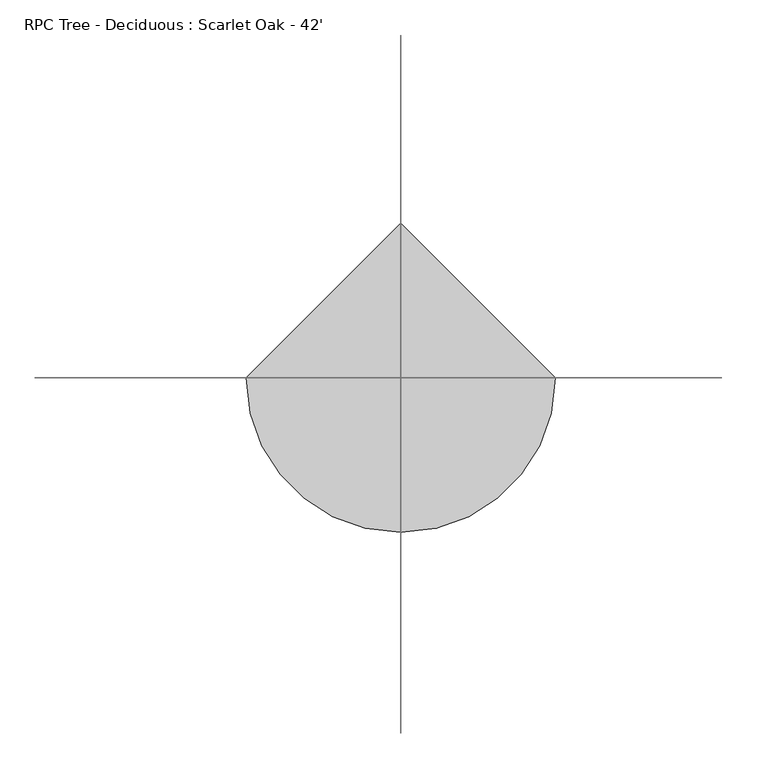
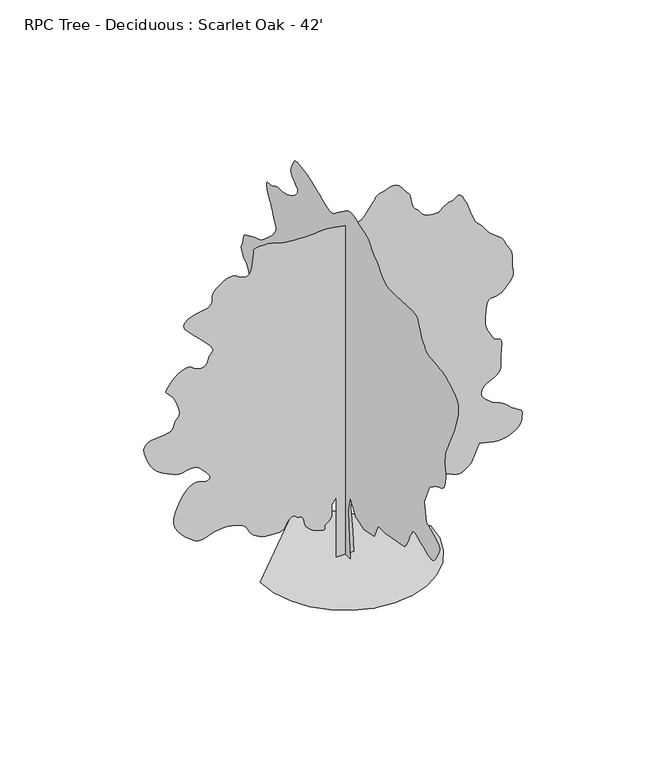
# IFC4 building model written with IfcOpenShell, lengths in millimetres: geographic element geometry, RPC Tree - Deciduous : Scarlet Oak - 42'.
# Revit data of these elements (continued)
# Type "RPC Tree - Deciduous : Scarlet Oak - 42'"
#   built-in parameter 1005198 = "{2, 15},{39, RPC-16-G0FB-J5PX-0LX6-U000-ST1L-LVER-AU},{1, 0},{1, 0},{2, 13},{1, 8},{5, Color},{1, 0},{1, 0},{3, 0.8},{3, 0.8},{3, 0.8},{1, 8},{7, BBoxMin},{1, 0},{1, 0},{1, 0},{1, 0},{1, 0},{1, 8},{7, BBoxMax},{1, 0},{1, 0},{1, 0},{1, 0},{1, 0},{2, 11},{9, RPCTypeId},{1, 0},{1, 0},{39, RPC-16-G0FB-J5PX-0LX6-U000-ST1L-LVER-AU},{1, 6},{14, RPCPlantHeight},{1, 0},{1, 0},{2, 42},{2, 11},{7, keyword},{1, 0},{1, 0},{34, :RPCs:Trees [General]:Geometry:RPC},{2, 11},{8, category},{1, 0},{1, 0},{15, Trees [General]},{2, 11},{12, LocalizedUID},{1, 0},{1, 0},{11, Scarlet_Oak},{2, 14},{6, Height},{1, 0},{1, 0},{2, 42},{1, 2},{16, Cast Reflections},{1, 0},{1, 0},{1, 0},{1, 2},{12, Cast Shadows},{1, 0},{1, 0},{1, 1},{1, 2},{9, Lock View},{1, 0},{1, 0},{1, 0},{1, 4},{5, ViewC},{1, 0},{1, 0},{1, 0},{21, assetlibrary_base.fbx},{1, 5},"
#   built-in parameter 1005195 = "RPC-16-G0FB-J5PX-0LX6-U000-ST1L-LVER-AU"
#   Type Comments = "Scarlet Oak"
#   Assembly Code = "G2050500"
#   Height = 42' - 0"
